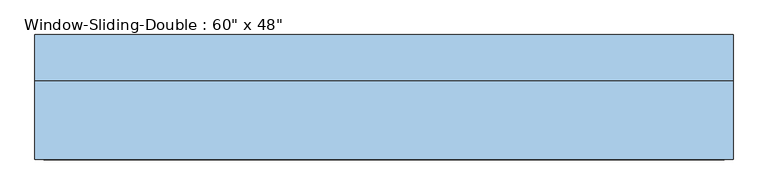
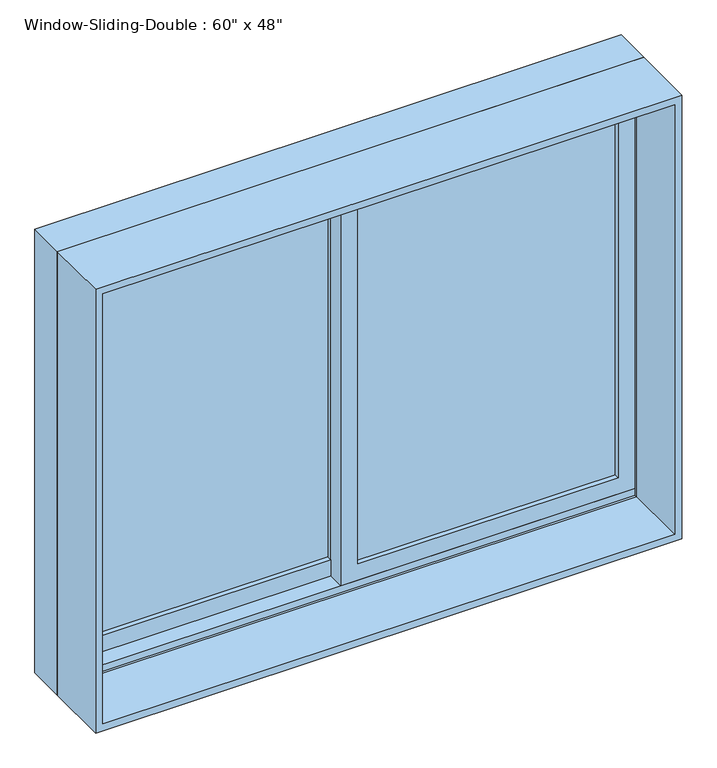
"""IFC4 building model written with IfcOpenShell, lengths in millimetres: window geometry."""

import ifcopenshell
import ifcopenshell.guid

model = None  # the IFC model being written
_history = None  # IfcOwnerHistory: only IFC2X3 demands one
_inside = {}  # id of a spatial element -> (the spatial element, [elements in it])
_under = {}  # id of a project, library or spatial element -> (it, [spatial elements below it])
_declared = {}  # id of a project -> (the project, [libraries it declares])
_typed = {}  # id of a type object -> (the type object, [elements of that type])
_made_of = {}  # id of a material, layer set ... -> (it, [elements and type objects made of it])


def new_model(schema):
    """Start an empty IFC model of exactly this schema.

    Asked for "IFC4X3", IfcOpenShell would pick the latest addendum, in which some entities
    have other attributes; the version numbers below select the first issue.
    IFC2X3 requires an IfcOwnerHistory on every rooted entity: one is made here for all.
    """
    global model, _history
    if schema == "IFC4X3":
        model = ifcopenshell.file(schema_version=(4, 3, 0, 0))
    else:
        model = ifcopenshell.file(schema=schema)
    _inside.clear()
    _under.clear()
    _declared.clear()
    _typed.clear()
    _made_of.clear()
    _history = None
    if model.schema == "IFC2X3":
        org = make("IfcOrganization", Name="unknown")
        user = make(
            "IfcPersonAndOrganization",
            ThePerson=make("IfcPerson", FamilyName="unknown"),
            TheOrganization=org,
        )
        app = make(
            "IfcApplication",
            ApplicationDeveloper=org,
            Version="unknown",
            ApplicationFullName="unknown",
            ApplicationIdentifier="unknown",
        )
        _history = make(
            "IfcOwnerHistory",
            OwningUser=user,
            OwningApplication=app,
            ChangeAction="ADDED",
            CreationDate=0,
        )
    return model


def make(cls, **values):
    """One entity of the class cls with the attributes given. An attribute that is None is left unset."""
    return model.create_entity(
        cls, **{name: value for name, value in values.items() if value is not None}
    )


def rooted(cls, **values):
    """An entity with a GlobalId (a new one), such as an element, a storey or a relation."""
    return make(cls, GlobalId=ifcopenshell.guid.new(), OwnerHistory=_history, **values)


def si_unit(unit_type, name, prefix=None):
    """IfcSIUnit, for example si_unit("LENGTHUNIT", "METRE", prefix="MILLI")."""
    return make("IfcSIUnit", UnitType=unit_type, Prefix=prefix, Name=name)


def assignment(units):
    """IfcUnitAssignment: the units of a project."""
    return None if units is None else make("IfcUnitAssignment", Units=units)


def point(xyz):
    """IfcCartesianPoint."""
    return None if xyz is None else make("IfcCartesianPoint", Coordinates=xyz)


def direction(xyz):
    """IfcDirection."""
    return None if xyz is None else make("IfcDirection", DirectionRatios=xyz)


def frame(location, z_axis=None, x_axis=None):
    """IfcAxis2Placement3D, a coordinate frame: its origin and axes. An axis left out is left unset."""
    return make(
        "IfcAxis2Placement3D",
        Location=point(location),
        Axis=direction(z_axis),
        RefDirection=direction(x_axis),
    )


def origin():
    """The frame at (0, 0, 0) with its axes left unset."""
    return frame((0.0, 0.0, 0.0))


def place(relative_to, where):
    """IfcLocalPlacement: puts the frame where relative to a parent placement (None: the world)."""
    return make(
        "IfcLocalPlacement", PlacementRelTo=relative_to, RelativePlacement=where
    )


def context(
    kind, dimensions, precision=None, world=None, true_north=None, identifier=None
):
    """IfcGeometricRepresentationContext, for example the 3D "Model" context."""
    return make(
        "IfcGeometricRepresentationContext",
        ContextIdentifier=identifier,
        ContextType=kind,
        CoordinateSpaceDimension=dimensions,
        Precision=precision,
        WorldCoordinateSystem=world,
        TrueNorth=true_north,
    )


def project(units=None, contexts=None):
    """IfcProject with its units and contexts."""
    return rooted(
        "IfcProject",
        Name="project",
        RepresentationContexts=contexts,
        UnitsInContext=assignment(units),
    )


def spatial(cls, under=None, at=None, **own):
    """A site, building, storey or space (cls), placed at a placement, below another one or the project."""
    s = rooted(cls, ObjectPlacement=at, **own)
    if under is not None:
        _under.setdefault(under.id(), (under, []))[1].append(s)
    return s


def polyline(points):
    """IfcPolyline through the points."""
    return make("IfcPolyline", Points=[point(p) for p in points])


def outline(outer, holes=None, kind="AREA"):
    """IfcArbitraryClosedProfileDef: a profile drawn as a closed curve; with holes, ...WithVoids."""
    if holes is None:
        return make("IfcArbitraryClosedProfileDef", ProfileType=kind, OuterCurve=outer)
    return make(
        "IfcArbitraryProfileDefWithVoids",
        ProfileType=kind,
        OuterCurve=outer,
        InnerCurves=holes,
    )


def extrude(swept, where, along, depth):
    """IfcExtrudedAreaSolid: the profile swept, set in the frame where, extruded along a direction by depth."""
    return make(
        "IfcExtrudedAreaSolid",
        SweptArea=swept,
        Position=where,
        ExtrudedDirection=direction(along),
        Depth=depth,
    )


def faces_of(points, faces, orient=None, outer=None):
    """IfcFace entities. A face is a list of loops; a loop is a list of indices into points, from 0.

    orient and outer hold one flag for each loop. By default every Orientation is true, the
    first loop of a face is its IfcFaceOuterBound and the others are IfcFaceBound.
    """
    made = []
    for i, loops in enumerate(faces):
        bounds = []
        for j, loop in enumerate(loops):
            is_outer = j == 0 if outer is None else outer[i][j]
            bounds.append(
                make(
                    "IfcFaceOuterBound" if is_outer else "IfcFaceBound",
                    Bound=make("IfcPolyLoop", Polygon=[points[k] for k in loop]),
                    Orientation=True if orient is None else orient[i][j],
                )
            )
        made.append(make("IfcFace", Bounds=bounds))
    return made


def faceted_brep(points, faces, orient=None, outer=None, voids=None):
    """IfcFacetedBrep: a solid bounded by flat faces; with voids (closed shells), ...WithVoids."""
    shared = [point(p) for p in points]
    hull = make("IfcClosedShell", CfsFaces=faces_of(shared, faces, orient, outer))
    if voids is None:
        return make("IfcFacetedBrep", Outer=hull)
    return make(
        "IfcFacetedBrepWithVoids",
        Outer=hull,
        Voids=[
            make(cls, CfsFaces=faces_of(shared, fs, o, b)) for cls, fs, o, b in voids
        ],
    )


def shape(context_of_items, identifier, shape_type, items):
    """IfcShapeRepresentation: the items that make up one representation, for example the "Body"."""
    return make(
        "IfcShapeRepresentation",
        ContextOfItems=context_of_items,
        RepresentationIdentifier=identifier,
        RepresentationType=shape_type,
        Items=items,
    )


def source(mapping_origin, context_of_items, identifier, shape_type, items):
    """IfcRepresentationMap: a shape defined once, which mapped items show again and again."""
    return make(
        "IfcRepresentationMap",
        MappingOrigin=mapping_origin,
        MappedRepresentation=shape(context_of_items, identifier, shape_type, items),
    )


def transform(
    local_origin,
    x_axis=None,
    y_axis=None,
    z_axis=None,
    scale=None,
    scale2=None,
    scale3=None,
    uniform=True,
):
    """IfcCartesianTransformationOperator3D, or its non-uniform kind. x_axis, y_axis, z_axis: its Axis1, 2, 3."""
    if uniform:
        return make(
            "IfcCartesianTransformationOperator3D",
            Axis1=direction(x_axis),
            Axis2=direction(y_axis),
            LocalOrigin=point(local_origin),
            Scale=scale,
            Axis3=direction(z_axis),
        )
    return make(
        "IfcCartesianTransformationOperator3DnonUniform",
        Axis1=direction(x_axis),
        Axis2=direction(y_axis),
        LocalOrigin=point(local_origin),
        Scale=scale,
        Axis3=direction(z_axis),
        Scale2=scale2,
        Scale3=scale3,
    )


def mapped(mapping_source, mapping_target):
    """IfcMappedItem: shows the shape of a source again, moved by a transform."""
    return make(
        "IfcMappedItem", MappingSource=mapping_source, MappingTarget=mapping_target
    )


def made_of(thing, what):
    """Note that an element or type object is made of a material, layer set ...; save() writes the relation."""
    if what is not None:
        _made_of.setdefault(what.id(), (what, []))[1].append(thing)
    return thing


def element(
    cls,
    number,
    at=None,
    inside=None,
    cuts=None,
    type_object=None,
    material=None,
    context=None,
    identifier="Body",
    shape_type=None,
    held_by="IfcProductDefinitionShape",
    body=None,
    shapes=None,
    **own,
):
    """One element of the class cls, such as IfcWall. Its Tag is "e" and its number.

    at: its placement. inside: the storey or other place that contains it. cuts: it is an
    opening in that element (IfcRelVoidsElement). A single representation is given by context,
    identifier, shape_type and body (its items); several are given by shapes. held_by: the class
    of the entity that holds the representations. save() writes the other relations.
    """
    e = rooted(cls, Tag="e%d" % number, ObjectPlacement=at, **own)
    if body is not None:
        shapes = [shape(context, identifier, shape_type, body)]
    if shapes is not None:
        e.Representation = make(held_by, Representations=shapes)
    if inside is not None:
        _inside.setdefault(inside.id(), (inside, []))[1].append(e)
    if cuts is not None:
        rooted(
            "IfcRelVoidsElement", RelatingBuildingElement=cuts, RelatedOpeningElement=e
        )
    if type_object is not None:
        _typed.setdefault(type_object.id(), (type_object, []))[1].append(e)
    return made_of(e, material)


def aggregate(whole, parts):
    """IfcRelAggregates: a whole, such as a stair, and the parts it consists of."""
    return rooted("IfcRelAggregates", RelatingObject=whole, RelatedObjects=parts)


def save(model, path):
    """Write the relations noted so far, then the file.

    IfcRelAggregates (storeys below a building ...), IfcRelContainedInSpatialStructure (elements
    in a storey), IfcRelDefinesByType, IfcRelAssociatesMaterial and IfcRelDeclares: one each for
    every whole, place, type object, material and project.
    """
    for whole, parts in _under.values():
        aggregate(whole, parts)
    for where, things in _inside.values():
        rooted(
            "IfcRelContainedInSpatialStructure",
            RelatedElements=things,
            RelatingStructure=where,
        )
    for kind, things in _typed.values():
        rooted("IfcRelDefinesByType", RelatedObjects=things, RelatingType=kind)
    for what, things in _made_of.values():
        rooted("IfcRelAssociatesMaterial", RelatedObjects=things, RelatingMaterial=what)
    for by, libraries in _declared.values():
        rooted("IfcRelDeclares", RelatingContext=by, RelatedDefinitions=libraries)
    model.write(path)


def window_af6eba4b(model_context):
    return source(origin(), model_context, "Body", "SolidModel", [
        extrude(outline(polyline([(952.5, 742.95), (2114.55, 742.95), (2114.55, -22.225), (952.5, -22.225), (952.5, 742.95)]), holes=[polyline([(996.95, 22.225), (2070.1, 22.225), (2070.1, 698.5), (996.95, 698.5), (996.95, 22.225)])]), frame((0.0, 46.99, 0.0), z_axis=(0.0, 1.0, 0.0), x_axis=(0.0, 0.0, 1.0)), (0.0, 0.0, 1.0), 44.45),
        extrude(outline(polyline([(933.45, -742.95), (933.45, 22.225), (2114.55, 22.225), (2114.55, -742.95), (933.45, -742.95)]), holes=[polyline([(2070.1, -22.225), (996.95, -22.225), (996.95, -698.5), (2070.1, -698.5), (2070.1, -22.225)])]), frame((0.0, 91.44, 0.0), z_axis=(0.0, 1.0, 0.0), x_axis=(0.0, 0.0, 1.0)), (0.0, 0.0, 1.0), 44.45),
        extrude(outline(polyline([(-22.225, 123.19), (-22.225, 116.84), (-698.5, 116.84), (-698.5, 123.19), (-22.225, 123.19)])), frame((0.0, 0.0, 996.95), z_axis=(0.0, 0.0, 1.0), x_axis=(1.0, 0.0, 0.0)), (0.0, 0.0, 1.0), 1073.15),
        extrude(outline(polyline([(-22.225, 110.49), (-22.225, 104.14), (-698.5, 104.14), (-698.5, 110.49), (-22.225, 110.49)])), frame((0.0, 0.0, 996.95), z_axis=(0.0, 0.0, 1.0), x_axis=(1.0, 0.0, 0.0)), (0.0, 0.0, 1.0), 1073.15),
        extrude(outline(polyline([(698.5, 78.74), (698.5, 72.39), (22.225, 72.39), (22.225, 78.74), (698.5, 78.74)])), frame((0.0, 0.0, 996.95), z_axis=(0.0, 0.0, 1.0), x_axis=(1.0, 0.0, 0.0)), (0.0, 0.0, 1.0), 1073.15),
        extrude(outline(polyline([(698.5, 66.04), (698.5, 59.69), (22.225, 59.69), (22.225, 66.04), (698.5, 66.04)])), frame((0.0, 0.0, 996.95), z_axis=(0.0, 0.0, 1.0), x_axis=(1.0, 0.0, 0.0)), (0.0, 0.0, 1.0), 1073.15),
        extrude(outline(polyline([(2133.6, -762.0), (914.4, -762.0), (914.4, 762.0), (2133.6, 762.0), (2133.6, -762.0)]), holes=[polyline([(2114.55, 742.95), (933.45, 742.95), (933.45, -742.95), (2114.55, -742.95), (2114.55, 742.95)])]), frame((0.0, -130.81, 0.0), z_axis=(0.0, 1.0, 0.0), x_axis=(0.0, 0.0, 1.0)), (0.0, 0.0, 1.0), 171.45),
        faceted_brep([(-762.0, 40.64, 914.4), (-762.0, 142.24, 914.4), (762.0, 142.24, 914.4), (762.0, 40.64, 914.4), (-721.0778905, 142.24, 2092.6778905), (-721.0778905, 135.89, 2092.6778905), (-721.0778905, 135.89, 933.45), (-721.0778905, 142.24, 933.45), (721.0778905, 135.89, 2092.6778905), (721.0778905, 135.89, 933.45), (742.95, 135.89, 933.45), (742.95, 135.89, 2114.55), (-742.95, 135.89, 2114.55), (-742.95, 135.89, 933.45), (-742.95, 40.64, 2114.55), (-742.95, 40.64, 933.45), (-742.95, 46.99, 933.45), (-742.95, 46.99, 952.5), (-742.95, 91.44, 952.5), (-742.95, 91.44, 933.45), (762.0, 40.64, 2133.6), (-762.0, 40.64, 2133.6), (742.95, 40.64, 2114.55), (742.95, 40.64, 933.45), (-762.0, 142.24, 2133.6), (762.0, 142.24, 2133.6), (721.0778905, 142.24, 933.45), (721.0778905, 142.24, 2092.6778905), (742.95, 91.44, 933.45), (742.95, 91.44, 952.5), (742.95, 46.99, 952.5), (742.95, 46.99, 933.45)], [[[0, 1, 2, 3]], [[4, 5, 6, 7]], [[5, 8, 9, 10, 11, 12, 13, 6]], [[12, 14, 15, 16, 17, 18, 19, 13]], [[0, 3, 20, 21], [22, 23, 15, 14]], [[24, 1, 0, 21]], [[2, 1, 24, 25], [4, 7, 26, 27]], [[5, 4, 27, 8]], [[12, 11, 22, 14]], [[21, 20, 25, 24]], [[8, 27, 26, 9]], [[22, 11, 10, 28, 29, 30, 31, 23]], [[20, 3, 2, 25]], [[26, 7, 6, 13, 19, 28, 10, 9]], [[28, 19, 18, 29]], [[29, 18, 17, 30]], [[30, 17, 16, 31]], [[15, 23, 31, 16]]]),
    ])


if __name__ == "__main__":
    model = new_model("IFC4")
    model_context = context("Model", 3, world=origin())
    ifc_project = project(units=[si_unit("LENGTHUNIT", "METRE", prefix="MILLI")], contexts=[model_context])
    site = spatial("IfcSite", under=ifc_project)
    building = spatial("IfcBuilding", under=site)
    placement = place(None, origin())
    window_shape = window_af6eba4b(model_context)
    element("IfcWindow", 1, ObjectType="Window-Sliding-Double : 60\" x 48\"", at=placement, inside=building, context=model_context, shape_type="MappedRepresentation", body=[
        mapped(window_shape, transform((0.0, 0.0, 0.0), x_axis=(1.0, 0.0, 0.0), y_axis=(0.0, 1.0, 0.0), z_axis=(0.0, 0.0, 1.0))),
    ])
    save(model, "model.ifc")

# Revit data of these elements
# Type "Window-Sliding-Double : 60\" x 48\""
#   Type Mark = "23"
#   Fire Rating = "0.5h"
#   Assembly Code = "B2020100"
#   Analytic Construction = "Double glazing - domestic"
#   Window Inset [instance default] = 0' - 0"
#   Wall Thickness [instance default] = 0' - 6"
#   Visual Light Transmittance = 0.81
#   Thermal Resistance (R) = 1.8146 (h·ft²·°F)/BTU
#   Solar Heat Gain Coefficient = 0.76
#   Muntin Width = 2' - 2 5/8"
#   Muntin Height = 3' - 6 1/4"
#   Interior Wall Closure [instance default] = 0' - 2 3/4"
#   Heat Transfer Coefficient (U) = 0.5511 BTU/(h·ft²·°F)
#   Frame Extension [instance default] = 0' - 0 1/4"
#   Exterior Wall Closure [instance default] = 0' - 1 1/4"
#   Rough Width = 5' - 0 1/2"
#   Rough Height = 4' - 0 1/2"
#   Height = 4' - 0"
#   Extension Jamb [instance default] = 0' - 2 3/4"
#   Default Sill Height = 3' - 0"
#   Width = 5' - 0"
#   Interior Trim Visibility [instance default] = yes
#   Indicator Visibility [instance default] = yes
#   Exterior Trim Visibility [instance default] = yes
#   Muntin Visibility = yes
#   Extension Jamb Visibility [instance default] = yes
#   Muntin Pattern = Muntin Pattern_2x2 : Muntin Pattern_2x2
#   Interior Trim Material = Wood - Stained
#   Interior Trim = Trim-Window-Interior-Flat : Picture Frame
#   Interior Frame Material = Wood - Stained
#   Glass Panel Material = Glass
#   Exterior Trim Material = Clad - White
#   Exterior Trim = Trim-Window-Exterior-Flat : with Sill
#   Exterior Frame Material = Clad - White
#   Wall Closure = (empty or 0)
# Element 1 (IfcWindow, "Window-Sliding-Double : 60\" x 48\"")
#   Wall Thickness = 0' - 10"
#   Extension Jamb = 0' - 6 3/4"
#   Materials on its faces: "Wood - Stained", "Glass", "Clad - White"
# Materials
#   "Wood - Stained": class "Wood", colour RGB 227 170 128, transparency 0, Cost = 0
#   "Glass": class "Glass", colour RGB 0 128 192, transparency 0.75, Description = "Soda Lime Glass", Cost = 0
#   "Clad - White": class "Wood", colour RGB 242 242 238, transparency 0, Cost = 0
